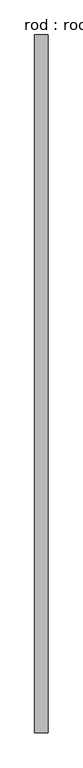
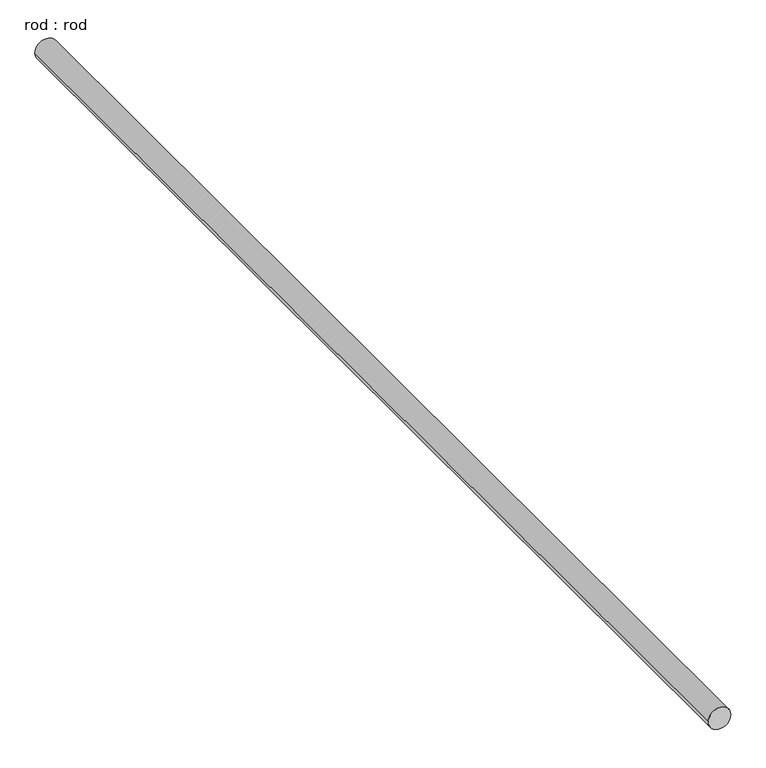
"""IFC4 building model written with IfcOpenShell, lengths in millimetres: proxy geometry, rod : rod."""

from ifc_helpers import new_model, si_unit, point, frame, frame_2d, origin, place, context, project, spatial, circle_curve, trimmed, segment, composite_curve, outline, extrude, source, transform, mapped, element, save


def rod_rod_8fa6ec7f(model_context):
    return source(origin(), model_context, "Body", "SweptSolid", [
        extrude(outline(composite_curve([segment(trimmed(circle_curve(frame_2d((0.0108462, 0.0)), 200.0), [point((0.0108462, 200.0))], [point((0.0108462, -200.0))], False, "CARTESIAN"), True, "CONTINUOUS"), segment(trimmed(circle_curve(frame_2d((0.0108462, 0.0)), 200.0), [point((0.0108462, -200.0))], [point((0.0108462, 200.0))], False, "CARTESIAN"), True, "CONTINUOUS")], self_intersect=False)), frame((0.0, -6252.6178935, 0.0), z_axis=(0.0, 1.0, 0.0), x_axis=(0.0, 0.0, 1.0)), (0.0, 0.0, 1.0), 20690.6930177),
    ])


if __name__ == "__main__":
    model = new_model("IFC4")
    model_context = context("Model", 3, world=origin())
    ifc_project = project(units=[si_unit("LENGTHUNIT", "METRE", prefix="MILLI")], contexts=[model_context])
    site = spatial("IfcSite", under=ifc_project)
    building = spatial("IfcBuilding", under=site)
    placement = place(None, origin())
    rod_rod_shape = rod_rod_8fa6ec7f(model_context)
    element("IfcBuildingElementProxy", 1, Name="rod : rod", ObjectType="rod : rod", at=placement, inside=building, context=model_context, shape_type="MappedRepresentation", body=[
        mapped(rod_rod_shape, transform((0.0, 0.0, 0.0), x_axis=(1.0, 0.0, 0.0), y_axis=(0.0, 1.0, 0.0), z_axis=(0.0, 0.0, 1.0))),
    ])
    save(model, "model.ifc")

# Revit data of these elements
# Type "rod : rod"
#   Default Elevation = 0
